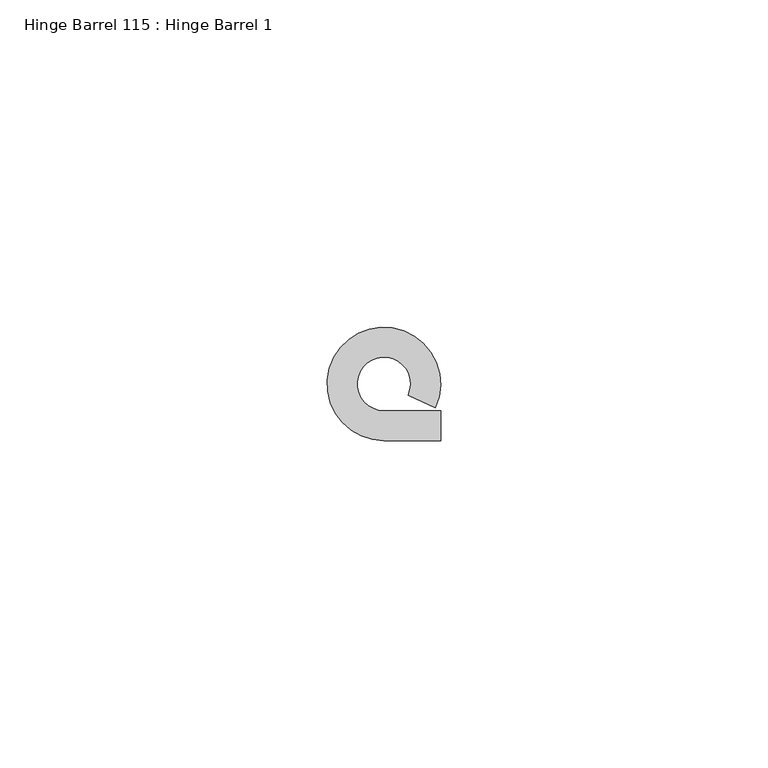
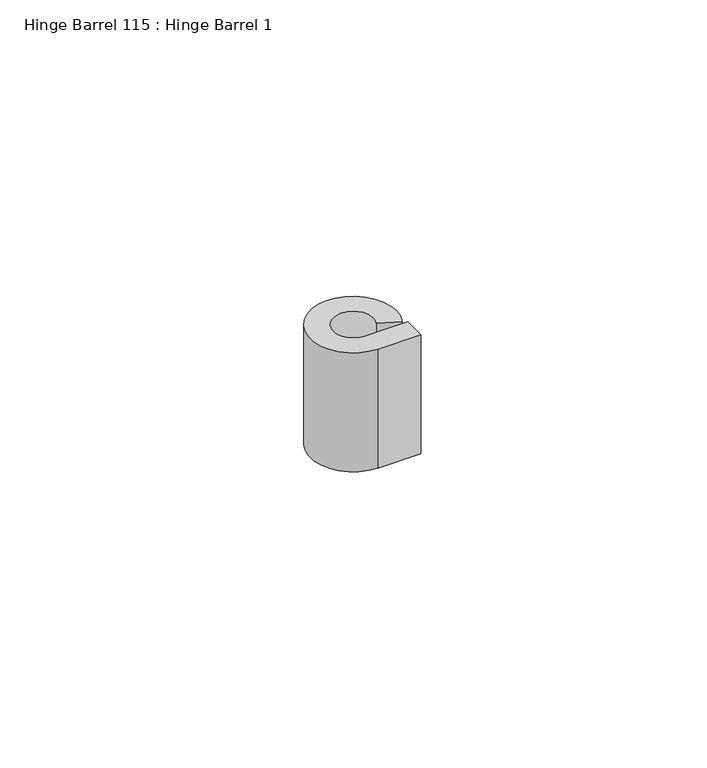
"""IFC4 building model written with IfcOpenShell, lengths in millimetres: proxy geometry, Hinge Barrel 115 : Hinge Barrel 1."""

import ifcopenshell
import ifcopenshell.guid

model = None  # the IFC model being written
_history = None  # IfcOwnerHistory: only IFC2X3 demands one
_inside = {}  # id of a spatial element -> (the spatial element, [elements in it])
_under = {}  # id of a project, library or spatial element -> (it, [spatial elements below it])
_declared = {}  # id of a project -> (the project, [libraries it declares])
_typed = {}  # id of a type object -> (the type object, [elements of that type])
_made_of = {}  # id of a material, layer set ... -> (it, [elements and type objects made of it])


def new_model(schema):
    """Start an empty IFC model of exactly this schema.

    Asked for "IFC4X3", IfcOpenShell would pick the latest addendum, in which some entities
    have other attributes; the version numbers below select the first issue.
    IFC2X3 requires an IfcOwnerHistory on every rooted entity: one is made here for all.
    """
    global model, _history
    if schema == "IFC4X3":
        model = ifcopenshell.file(schema_version=(4, 3, 0, 0))
    else:
        model = ifcopenshell.file(schema=schema)
    _inside.clear()
    _under.clear()
    _declared.clear()
    _typed.clear()
    _made_of.clear()
    _history = None
    if model.schema == "IFC2X3":
        org = make("IfcOrganization", Name="unknown")
        user = make(
            "IfcPersonAndOrganization",
            ThePerson=make("IfcPerson", FamilyName="unknown"),
            TheOrganization=org,
        )
        app = make(
            "IfcApplication",
            ApplicationDeveloper=org,
            Version="unknown",
            ApplicationFullName="unknown",
            ApplicationIdentifier="unknown",
        )
        _history = make(
            "IfcOwnerHistory",
            OwningUser=user,
            OwningApplication=app,
            ChangeAction="ADDED",
            CreationDate=0,
        )
    return model


def make(cls, **values):
    """One entity of the class cls with the attributes given. An attribute that is None is left unset."""
    return model.create_entity(
        cls, **{name: value for name, value in values.items() if value is not None}
    )


def rooted(cls, **values):
    """An entity with a GlobalId (a new one), such as an element, a storey or a relation."""
    return make(cls, GlobalId=ifcopenshell.guid.new(), OwnerHistory=_history, **values)


def si_unit(unit_type, name, prefix=None):
    """IfcSIUnit, for example si_unit("LENGTHUNIT", "METRE", prefix="MILLI")."""
    return make("IfcSIUnit", UnitType=unit_type, Prefix=prefix, Name=name)


def assignment(units):
    """IfcUnitAssignment: the units of a project."""
    return None if units is None else make("IfcUnitAssignment", Units=units)


def point(xyz):
    """IfcCartesianPoint."""
    return None if xyz is None else make("IfcCartesianPoint", Coordinates=xyz)


def direction(xyz):
    """IfcDirection."""
    return None if xyz is None else make("IfcDirection", DirectionRatios=xyz)


def frame(location, z_axis=None, x_axis=None):
    """IfcAxis2Placement3D, a coordinate frame: its origin and axes. An axis left out is left unset."""
    return make(
        "IfcAxis2Placement3D",
        Location=point(location),
        Axis=direction(z_axis),
        RefDirection=direction(x_axis),
    )


def frame_2d(location, x_axis=None):
    """IfcAxis2Placement2D, a coordinate frame in the plane: its origin and x axis."""
    return make(
        "IfcAxis2Placement2D", Location=point(location), RefDirection=direction(x_axis)
    )


def origin():
    """The frame at (0, 0, 0) with its axes left unset."""
    return frame((0.0, 0.0, 0.0))


def place(relative_to, where):
    """IfcLocalPlacement: puts the frame where relative to a parent placement (None: the world)."""
    return make(
        "IfcLocalPlacement", PlacementRelTo=relative_to, RelativePlacement=where
    )


def context(
    kind, dimensions, precision=None, world=None, true_north=None, identifier=None
):
    """IfcGeometricRepresentationContext, for example the 3D "Model" context."""
    return make(
        "IfcGeometricRepresentationContext",
        ContextIdentifier=identifier,
        ContextType=kind,
        CoordinateSpaceDimension=dimensions,
        Precision=precision,
        WorldCoordinateSystem=world,
        TrueNorth=true_north,
    )


def project(units=None, contexts=None):
    """IfcProject with its units and contexts."""
    return rooted(
        "IfcProject",
        Name="project",
        RepresentationContexts=contexts,
        UnitsInContext=assignment(units),
    )


def spatial(cls, under=None, at=None, **own):
    """A site, building, storey or space (cls), placed at a placement, below another one or the project."""
    s = rooted(cls, ObjectPlacement=at, **own)
    if under is not None:
        _under.setdefault(under.id(), (under, []))[1].append(s)
    return s


def polyline(points):
    """IfcPolyline through the points."""
    return make("IfcPolyline", Points=[point(p) for p in points])


def circle_curve(where, radius):
    """IfcCircle in the frame where."""
    return make("IfcCircle", Position=where, Radius=radius)


def trimmed(basis, trim1, trim2, sense, master):
    """IfcTrimmedCurve: the piece of a basis curve between two trims."""
    return make(
        "IfcTrimmedCurve",
        BasisCurve=basis,
        Trim1=trim1,
        Trim2=trim2,
        SenseAgreement=sense,
        MasterRepresentation=master,
    )


def segment(curve, same_sense, transition):
    """IfcCompositeCurveSegment."""
    return make(
        "IfcCompositeCurveSegment",
        Transition=transition,
        SameSense=same_sense,
        ParentCurve=curve,
    )


def composite_curve(segments, self_intersect=None):
    """IfcCompositeCurve: segments joined end to end."""
    return make("IfcCompositeCurve", Segments=segments, SelfIntersect=self_intersect)


def outline(outer, holes=None, kind="AREA"):
    """IfcArbitraryClosedProfileDef: a profile drawn as a closed curve; with holes, ...WithVoids."""
    if holes is None:
        return make("IfcArbitraryClosedProfileDef", ProfileType=kind, OuterCurve=outer)
    return make(
        "IfcArbitraryProfileDefWithVoids",
        ProfileType=kind,
        OuterCurve=outer,
        InnerCurves=holes,
    )


def extrude(swept, where, along, depth):
    """IfcExtrudedAreaSolid: the profile swept, set in the frame where, extruded along a direction by depth."""
    return make(
        "IfcExtrudedAreaSolid",
        SweptArea=swept,
        Position=where,
        ExtrudedDirection=direction(along),
        Depth=depth,
    )


def shape(context_of_items, identifier, shape_type, items):
    """IfcShapeRepresentation: the items that make up one representation, for example the "Body"."""
    return make(
        "IfcShapeRepresentation",
        ContextOfItems=context_of_items,
        RepresentationIdentifier=identifier,
        RepresentationType=shape_type,
        Items=items,
    )


def source(mapping_origin, context_of_items, identifier, shape_type, items):
    """IfcRepresentationMap: a shape defined once, which mapped items show again and again."""
    return make(
        "IfcRepresentationMap",
        MappingOrigin=mapping_origin,
        MappedRepresentation=shape(context_of_items, identifier, shape_type, items),
    )


def transform(
    local_origin,
    x_axis=None,
    y_axis=None,
    z_axis=None,
    scale=None,
    scale2=None,
    scale3=None,
    uniform=True,
):
    """IfcCartesianTransformationOperator3D, or its non-uniform kind. x_axis, y_axis, z_axis: its Axis1, 2, 3."""
    if uniform:
        return make(
            "IfcCartesianTransformationOperator3D",
            Axis1=direction(x_axis),
            Axis2=direction(y_axis),
            LocalOrigin=point(local_origin),
            Scale=scale,
            Axis3=direction(z_axis),
        )
    return make(
        "IfcCartesianTransformationOperator3DnonUniform",
        Axis1=direction(x_axis),
        Axis2=direction(y_axis),
        LocalOrigin=point(local_origin),
        Scale=scale,
        Axis3=direction(z_axis),
        Scale2=scale2,
        Scale3=scale3,
    )


def mapped(mapping_source, mapping_target):
    """IfcMappedItem: shows the shape of a source again, moved by a transform."""
    return make(
        "IfcMappedItem", MappingSource=mapping_source, MappingTarget=mapping_target
    )


def made_of(thing, what):
    """Note that an element or type object is made of a material, layer set ...; save() writes the relation."""
    if what is not None:
        _made_of.setdefault(what.id(), (what, []))[1].append(thing)
    return thing


def element(
    cls,
    number,
    at=None,
    inside=None,
    cuts=None,
    type_object=None,
    material=None,
    context=None,
    identifier="Body",
    shape_type=None,
    held_by="IfcProductDefinitionShape",
    body=None,
    shapes=None,
    **own,
):
    """One element of the class cls, such as IfcWall. Its Tag is "e" and its number.

    at: its placement. inside: the storey or other place that contains it. cuts: it is an
    opening in that element (IfcRelVoidsElement). A single representation is given by context,
    identifier, shape_type and body (its items); several are given by shapes. held_by: the class
    of the entity that holds the representations. save() writes the other relations.
    """
    e = rooted(cls, Tag="e%d" % number, ObjectPlacement=at, **own)
    if body is not None:
        shapes = [shape(context, identifier, shape_type, body)]
    if shapes is not None:
        e.Representation = make(held_by, Representations=shapes)
    if inside is not None:
        _inside.setdefault(inside.id(), (inside, []))[1].append(e)
    if cuts is not None:
        rooted(
            "IfcRelVoidsElement", RelatingBuildingElement=cuts, RelatedOpeningElement=e
        )
    if type_object is not None:
        _typed.setdefault(type_object.id(), (type_object, []))[1].append(e)
    return made_of(e, material)


def aggregate(whole, parts):
    """IfcRelAggregates: a whole, such as a stair, and the parts it consists of."""
    return rooted("IfcRelAggregates", RelatingObject=whole, RelatedObjects=parts)


def save(model, path):
    """Write the relations noted so far, then the file.

    IfcRelAggregates (storeys below a building ...), IfcRelContainedInSpatialStructure (elements
    in a storey), IfcRelDefinesByType, IfcRelAssociatesMaterial and IfcRelDeclares: one each for
    every whole, place, type object, material and project.
    """
    for whole, parts in _under.values():
        aggregate(whole, parts)
    for where, things in _inside.values():
        rooted(
            "IfcRelContainedInSpatialStructure",
            RelatedElements=things,
            RelatingStructure=where,
        )
    for kind, things in _typed.values():
        rooted("IfcRelDefinesByType", RelatedObjects=things, RelatingType=kind)
    for what, things in _made_of.values():
        rooted("IfcRelAssociatesMaterial", RelatedObjects=things, RelatingMaterial=what)
    for by, libraries in _declared.values():
        rooted("IfcRelDeclares", RelatingContext=by, RelatedDefinitions=libraries)
    model.write(path)


def hinge_barrel_115_hinge_barrel_1_81794a76(model_context):
    return source(origin(), model_context, "Body", "SweptSolid", [
        extrude(outline(composite_curve([segment(polyline([(587323.2214739, -534104.7943841), (587327.7934739, -534104.7943841), (587327.7934739, -534109.3584466), (587319.1320739, -534109.3584466)]), True, "CONTINUOUS"), segment(trimmed(circle_curve(frame_2d((587319.1320739, -534100.7049841)), 8.6534625), [point((587319.1320739, -534109.3584466))], [point((587326.986084, -534104.3377433))], False, "CARTESIAN"), True, "CONTINUOUS"), segment(polyline([(587326.986084, -534104.3377433), (587322.8436736, -534102.421731)]), True, "CONTINUOUS"), segment(trimmed(circle_curve(frame_2d((587319.1320739, -534100.7049841)), 4.0894), [point((587322.8436736, -534102.421731))], [point((587319.1320739, -534104.7943841))], True, "CARTESIAN"), True, "CONTINUOUS"), segment(polyline([(587319.1320739, -534104.7943841), (587323.2214739, -534104.7943841)]), True, "CONTINUOUS")], self_intersect=False)), frame((0.0, 0.0, 1936.75), z_axis=(0.0, 0.0, 1.0), x_axis=(1.0, 0.0, 0.0)), (0.0, 0.0, 1.0), 25.4),
    ])


if __name__ == "__main__":
    model = new_model("IFC4")
    model_context = context("Model", 3, world=origin())
    ifc_project = project(units=[si_unit("LENGTHUNIT", "METRE", prefix="MILLI")], contexts=[model_context])
    site = spatial("IfcSite", under=ifc_project)
    building = spatial("IfcBuilding", under=site)
    placement = place(None, origin())
    hinge_barrel_115_hinge_barrel_1_shape = hinge_barrel_115_hinge_barrel_1_81794a76(model_context)
    element("IfcBuildingElementProxy", 1, Name="Hinge Barrel 115 : Hinge Barrel 1", ObjectType="Hinge Barrel 115 : Hinge Barrel 1", at=placement, inside=building, context=model_context, shape_type="MappedRepresentation", body=[
        mapped(hinge_barrel_115_hinge_barrel_1_shape, transform((0.0, 0.0, 0.0), x_axis=(1.0, 0.0, 0.0), y_axis=(0.0, 1.0, 0.0), z_axis=(0.0, 0.0, 1.0))),
    ])
    save(model, "model.ifc")

# Revit data of these elements
# Element 1 (IfcBuildingElementProxy, "Hinge Barrel 115 : Hinge Barrel 1")
#   Materials on its faces: "6\"X6\" WELD-ON STL BUTT HINGE"
# Materials
#   "6\"X6\" WELD-ON STL BUTT HINGE": class "Metal", colour RGB 189 187 185, transparency 0, Description = "Carbon steel", Cost = 0
